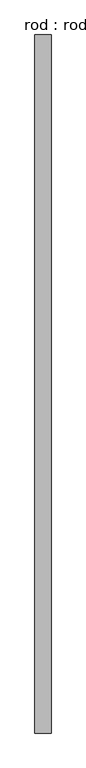
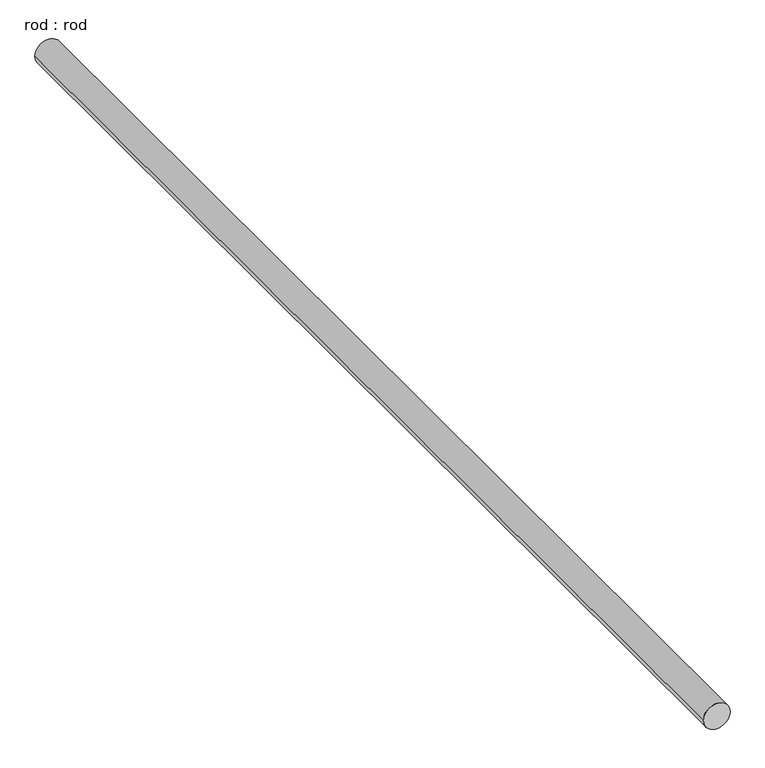
"""IFC4 building model written with IfcOpenShell, lengths in millimetres: proxy geometry, rod : rod."""

from ifc_helpers import new_model, si_unit, point, frame, frame_2d, origin, place, context, project, spatial, circle_curve, trimmed, segment, composite_curve, outline, extrude, source, transform, mapped, element, save


def rod_rod_9104e5f4(model_context):
    return source(origin(), model_context, "Body", "SweptSolid", [
        extrude(outline(composite_curve([segment(trimmed(circle_curve(frame_2d((0.0108462, 0.0)), 200.0), [point((0.0108462, 200.0))], [point((0.0108462, -200.0))], False, "CARTESIAN"), True, "CONTINUOUS"), segment(trimmed(circle_curve(frame_2d((0.0108462, 0.0)), 200.0), [point((0.0108462, -200.0))], [point((0.0108462, 200.0))], False, "CARTESIAN"), True, "CONTINUOUS")], self_intersect=False)), frame((0.0, -4573.9380513, 0.0), z_axis=(0.0, 1.0, 0.0), x_axis=(0.0, 0.0, 1.0)), (0.0, 0.0, 1.0), 17333.3333333),
    ])


if __name__ == "__main__":
    model = new_model("IFC4")
    model_context = context("Model", 3, world=origin())
    ifc_project = project(units=[si_unit("LENGTHUNIT", "METRE", prefix="MILLI")], contexts=[model_context])
    site = spatial("IfcSite", under=ifc_project)
    building = spatial("IfcBuilding", under=site)
    placement = place(None, origin())
    rod_rod_shape = rod_rod_9104e5f4(model_context)
    element("IfcBuildingElementProxy", 1, Name="rod : rod", ObjectType="rod : rod", at=placement, inside=building, context=model_context, shape_type="MappedRepresentation", body=[
        mapped(rod_rod_shape, transform((0.0, 0.0, 0.0), x_axis=(1.0, 0.0, 0.0), y_axis=(0.0, 1.0, 0.0), z_axis=(0.0, 0.0, 1.0))),
    ])
    save(model, "model.ifc")

# Revit data of these elements
# Type "rod : rod"
#   Default Elevation = 0
